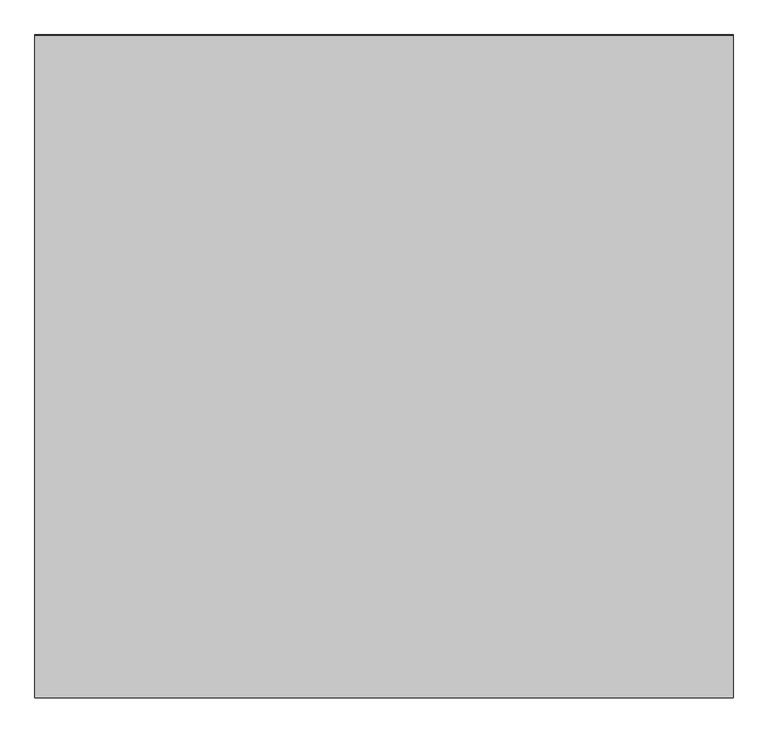
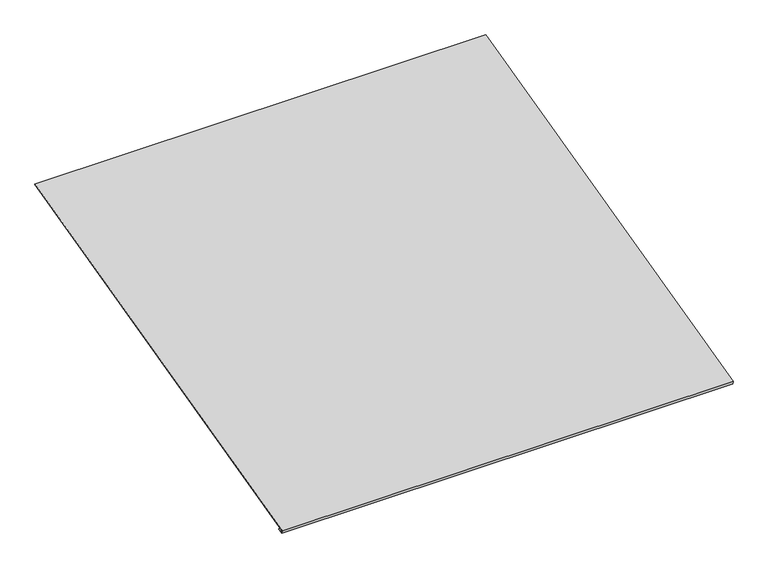
"""IFC4 building model written with IfcOpenShell, lengths in millimetres: proxy geometry, Gutter @ Roof : Gutter @ Roof."""

from ifc_helpers import new_model, si_unit, frame, origin, place, context, project, spatial, polyline, outline, extrude, source, transform, mapped, element, save


def generic_models_0034b9cc(model_context):
    return source(origin(), model_context, "Body", "SweptSolid", [
        extrude(outline(polyline([(-5229.4752646, 42838.5904488), (-5251.4724556, 42832.9050044), (-5254.9401206, 42846.7756645), (-3355.5497665, 43321.6232532), (-3354.9337261, 43319.1590912), (-5251.8611444, 42844.9272365), (-5249.5596959, 42836.0228487), (-5230.1108718, 42841.0496364), (-5229.4752646, 42838.5904488)])), frame((12382.7678845, 0.0, 0.0), z_axis=(1.0, 0.0, 0.0), x_axis=(0.0, 1.0, 0.0)), (0.0, 0.0, 1.0), 2000.25),
    ])


if __name__ == "__main__":
    model = new_model("IFC4")
    model_context = context("Model", 3, world=origin())
    ifc_project = project(units=[si_unit("LENGTHUNIT", "METRE", prefix="MILLI")], contexts=[model_context])
    site = spatial("IfcSite", under=ifc_project)
    building = spatial("IfcBuilding", under=site)
    placement = place(None, origin())
    generic_models_shape = generic_models_0034b9cc(model_context)
    element("IfcBuildingElementProxy", 1, Name="Gutter @ Roof : Gutter @ Roof", ObjectType="Gutter @ Roof : Gutter @ Roof", at=placement, inside=building, context=model_context, shape_type="MappedRepresentation", body=[
        mapped(generic_models_shape, transform((0.0, 0.0, 0.0), x_axis=(1.0, 0.0, 0.0), y_axis=(0.0, 1.0, 0.0), z_axis=(0.0, 0.0, 1.0))),
    ])
    save(model, "model.ifc")

# Revit data of these elements
# Project information
#   Issued Date 1 = "0/00/2018 - City of Newport Beach"
#   IfcSite GUID = "3hCLsSIbaHwOLX093rt3ko"
#   IfcBuilding GUID = "3hCN2YIbaHwOLX093rt3ko"
#   IfcProject GUID = "7043067b_ee86_4e71_a94"
#   NameOverride = "Default Site"
#   Project Issue Date = "Issue Date"
#   Project Status = "Project Status"
#   Client Name = "xxx"
#   Project Address = "xxx"
#   Project Name = "STAUDENMEIER RESIDENCE"
# Type "Gutter @ Roof : Gutter @ Roof"
#   NameOverride = "Gutter @ Roof"
# Element 1 (IfcBuildingElementProxy, "Gutter @ Roof : Gutter @ Roof")
#   Materials on its faces: "CONT. SEAMLESS 16 GA COPPER BRAKE METAL GUTTER"
# Materials
#   "CONT. SEAMLESS 16 GA COPPER BRAKE METAL GUTTER": class "Unassigned", colour RGB 128 128 128, transparency 0
